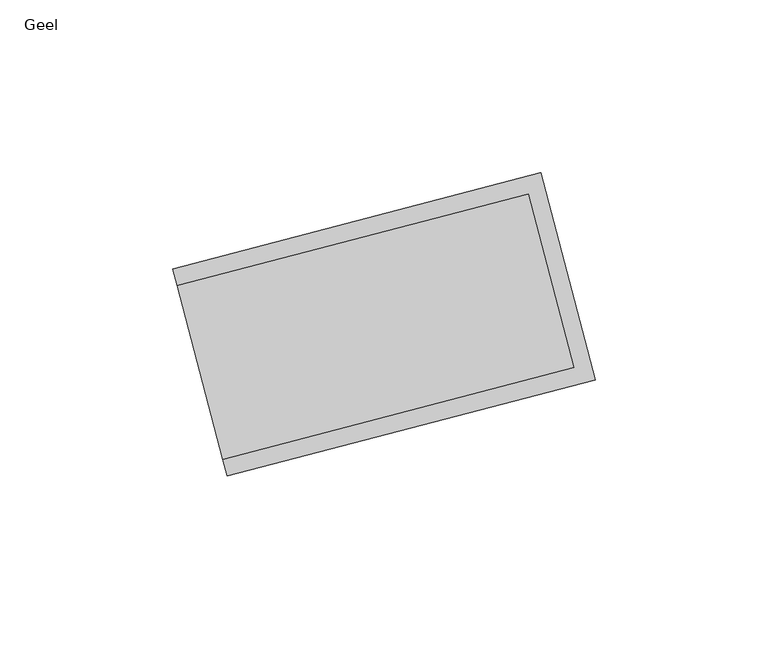
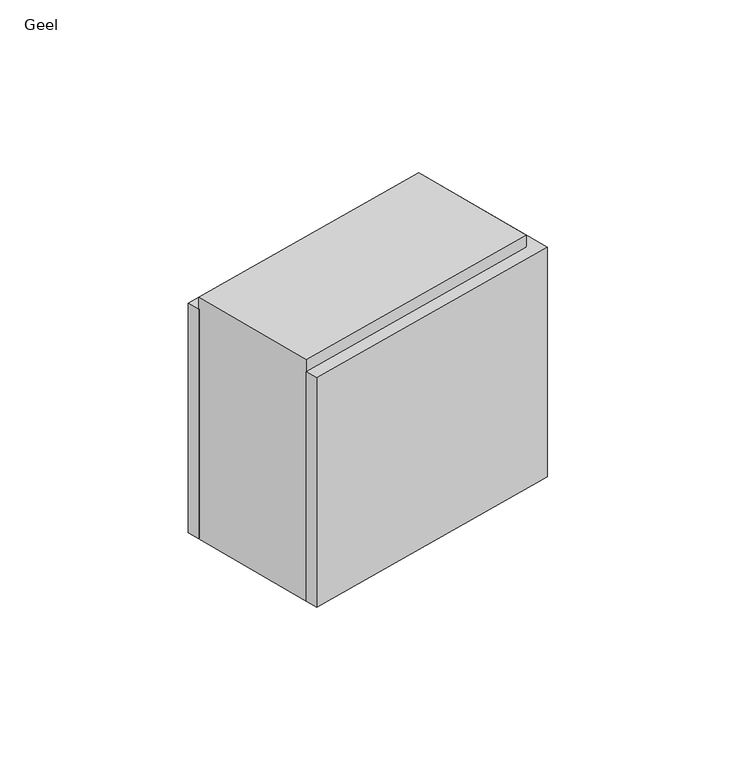
"""IFC4 building model written with IfcOpenShell, lengths in millimetres: proxy geometry, 00_GMA_steen_versie_6 : Geel."""

from ifc_helpers import new_model, si_unit, origin, origin_with_axes, place, context, project, spatial, polyline, outline, extrude, source, transform, mapped, element, save


def geel_a5fc7152(model_context):
    return source(origin(), model_context, "Body", "SweptSolid", [
        extrude(outline(polyline([(131.1871262, 51.8695461), (24.8461542, 24.0369432), (23.5801491, 28.8740117), (125.0840527, 55.4406095), (111.9430518, 105.6488784), (10.4391482, 79.0822806), (9.1731432, 83.919349), (115.5141152, 111.7519519), (131.1871262, 51.8695461)])), origin_with_axes(), (0.0, 0.0, 1.0), 95.0),
        extrude(outline(polyline([(111.9430518, 105.6488784), (125.0840527, 55.4406095), (23.5801491, 28.8740117), (10.4391482, 79.0822806), (111.9430518, 105.6488784)])), origin_with_axes(), (0.0, 0.0, 1.0), 100.0),
    ])


if __name__ == "__main__":
    model = new_model("IFC4")
    model_context = context("Model", 3, world=origin())
    ifc_project = project(units=[si_unit("LENGTHUNIT", "METRE", prefix="MILLI")], contexts=[model_context])
    site = spatial("IfcSite", under=ifc_project)
    building = spatial("IfcBuilding", under=site)
    placement = place(None, origin())
    geel_shape = geel_a5fc7152(model_context)
    element("IfcBuildingElementProxy", 1, Name="00_GMA_steen_versie_6 : Geel", ObjectType="00_GMA_steen_versie_6 : Geel", at=placement, inside=building, context=model_context, shape_type="MappedRepresentation", body=[
        mapped(geel_shape, transform((0.0, 0.0, 0.0), x_axis=(1.0, 0.0, 0.0), y_axis=(0.0, 1.0, 0.0), z_axis=(0.0, 0.0, 1.0))),
    ])
    save(model, "model.ifc")

# Revit data of these elements
# Type "00_GMA_steen_versie_6 : Geel"
#   Voegdikte = 95 mm
#   VoegTovSteen = -5 mm
#   StootvoegLinksHalfOnder [instance default] = 5 mm
#   StootvoegLinksHalfBoven [instance default] = 5 mm
#   StootVoegRechtsHalfOnder [instance default] = 5 mm
#   StootVoegRechtsHalfBoven [instance default] = 5 mm
#   StootVoegBreedteRechts [instance default] = 10 mm
#   StootVoegBreedteLinks [instance default] = 10 mm
#   Steendikte = 100 mm
#   LintVoegOnderHalf [instance default] = 0 mm
#   LintVoegOnder [instance default] = 0 mm
#   LintVoegBovenHalf [instance default] = 5 mm
#   LintVoegBoven [instance default] = 10 mm
#   materiaal = 21_steen_geel
#   MateriaalVoeg = 20_voeg
#   Default Elevation = 0
# Element 1 (IfcBuildingElementProxy, "00_GMA_steen_versie_6 : Geel")
#   StootvoegLinksHalfOnder = 0 mm
#   StootvoegLinksHalfBoven = 0 mm
#   StootVoegBreedteLinks = 0 mm
#   LintVoegOnderHalf = 5 mm
#   LintVoegOnder = 10 mm
#   Materials on its faces: "20_voeg", "21_steen_geel"
# Materials
#   "21_steen_geel": class "Unassigned", colour RGB 202 202 0, transparency 0, Cost = 0
#   "20_voeg": class "Concrete", colour RGB 86 86 86, transparency 0, Manufacturer = "RevitGG", URL = "www.revitgg.nl", Description = "zandcement, generiek materiaal", Cost = 0
